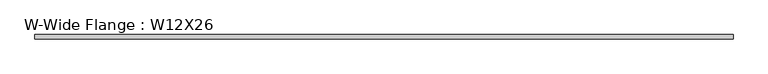
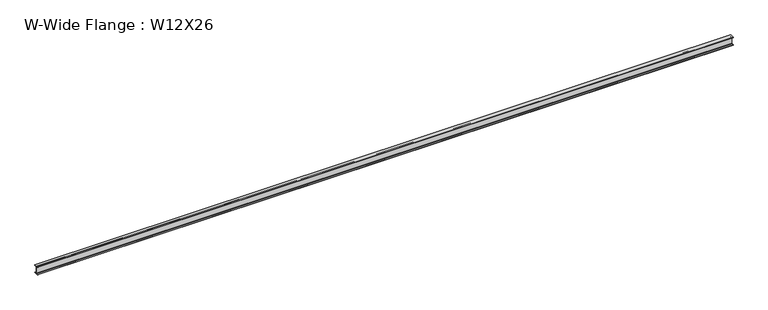
"""IFC4 building model written with IfcOpenShell, lengths in millimetres: beam geometry, W-Wide Flange : W12X26."""

from ifc_helpers import new_model, si_unit, point, frame, frame_2d, origin, place, context, project, spatial, polyline, circle_curve, trimmed, segment, composite_curve, outline, extrude, source, transform, mapped, element, save


def w_wide_flange_w12x26_1b2d4b26(model_context):
    return source(origin(), model_context, "Body", "SweptSolid", [
        extrude(outline(composite_curve([segment(polyline([(82.4011719, -145.5539063), (82.4011719, -155.178125), (-82.4011719, -155.178125), (-82.4011719, -145.5539063), (-20.2902344, -145.5539063)]), True, "CONTINUOUS"), segment(trimmed(circle_curve(frame_2d((-20.2902344, -128.190625)), 17.3632812), [point((-20.2902344, -145.5539063))], [point((-2.9269531, -128.190625))], True, "CARTESIAN"), True, "CONTINUOUS"), segment(polyline([(-2.9269531, -128.190625), (-2.9269531, 128.190625)]), True, "CONTINUOUS"), segment(trimmed(circle_curve(frame_2d((-20.2902344, 128.190625)), 17.3632812), [point((-2.9269531, 128.190625))], [point((-20.2902344, 145.5539062))], True, "CARTESIAN"), True, "CONTINUOUS"), segment(polyline([(-20.2902344, 145.5539062), (-82.4011719, 145.5539062), (-82.4011719, 155.178125), (82.4011719, 155.178125), (82.4011719, 145.5539062), (20.2902344, 145.5539062)]), True, "CONTINUOUS"), segment(trimmed(circle_curve(frame_2d((20.2902344, 128.190625)), 17.3632812), [point((20.2902344, 145.5539062))], [point((2.9269531, 128.190625))], True, "CARTESIAN"), True, "CONTINUOUS"), segment(polyline([(2.9269531, 128.190625), (2.9269531, -128.190625)]), True, "CONTINUOUS"), segment(trimmed(circle_curve(frame_2d((20.2902344, -128.190625)), 17.3632812), [point((2.9269531, -128.190625))], [point((20.2902344, -145.5539063))], True, "CARTESIAN"), True, "CONTINUOUS"), segment(polyline([(20.2902344, -145.5539063), (82.4011719, -145.5539063)]), True, "CONTINUOUS")], self_intersect=False)), frame((-13301.6625, 0.0, 0.0), z_axis=(1.0, 0.0, 0.0), x_axis=(0.0, 1.0, 0.0)), (0.0, 0.0, 1.0), 26712.8625),
    ])


if __name__ == "__main__":
    model = new_model("IFC4")
    model_context = context("Model", 3, world=origin())
    ifc_project = project(units=[si_unit("LENGTHUNIT", "METRE", prefix="MILLI")], contexts=[model_context])
    site = spatial("IfcSite", under=ifc_project)
    building = spatial("IfcBuilding", under=site)
    placement = place(None, origin())
    w_wide_flange_w12x26_shape = w_wide_flange_w12x26_1b2d4b26(model_context)
    element("IfcBeam", 1, ObjectType="W-Wide Flange : W12X26", at=placement, inside=building, context=model_context, shape_type="MappedRepresentation", body=[
        mapped(w_wide_flange_w12x26_shape, transform((0.0, 0.0, 0.0), x_axis=(1.0, 0.0, 0.0), y_axis=(0.0, 1.0, 0.0), z_axis=(0.0, 0.0, 1.0))),
    ])
    save(model, "model.ifc")

# Revit data of these elements
# Type "W-Wide Flange : W12X26"
#   Assembly Code = "B10"
#   W = 26
#   Length [instance default] = 5' - 0"
#   bf = 0' - 6 125/256"
#   d = 1' - 0 7/32"
#   k = 0' - 1 1/16"
#   k2 = 0' - 0 175/256"
#   tf = 0' - 0 97/256"
#   tw = 0' - 0 59/256"
#   A = 0.053125 SF
#   Structural Material [instance default] = none
